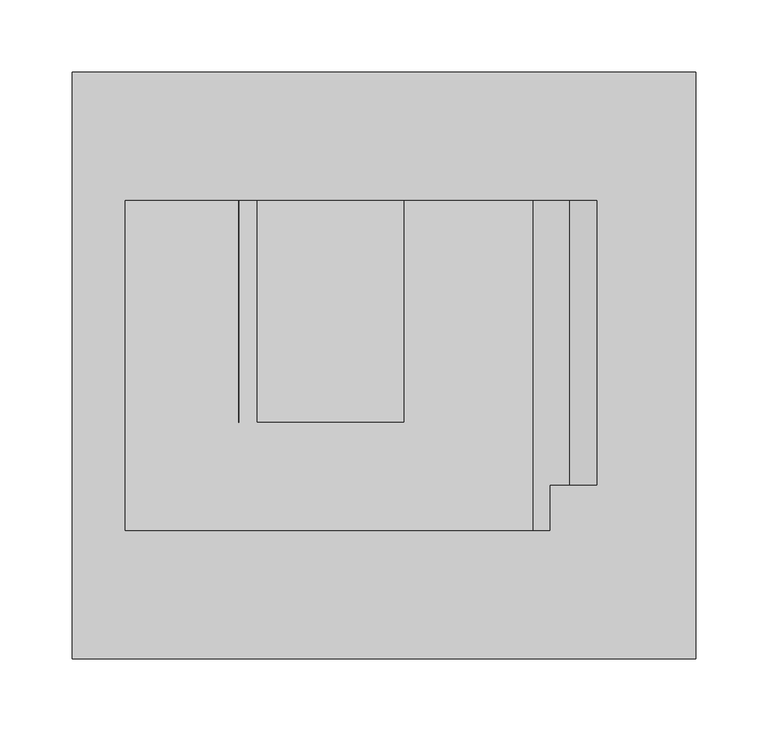
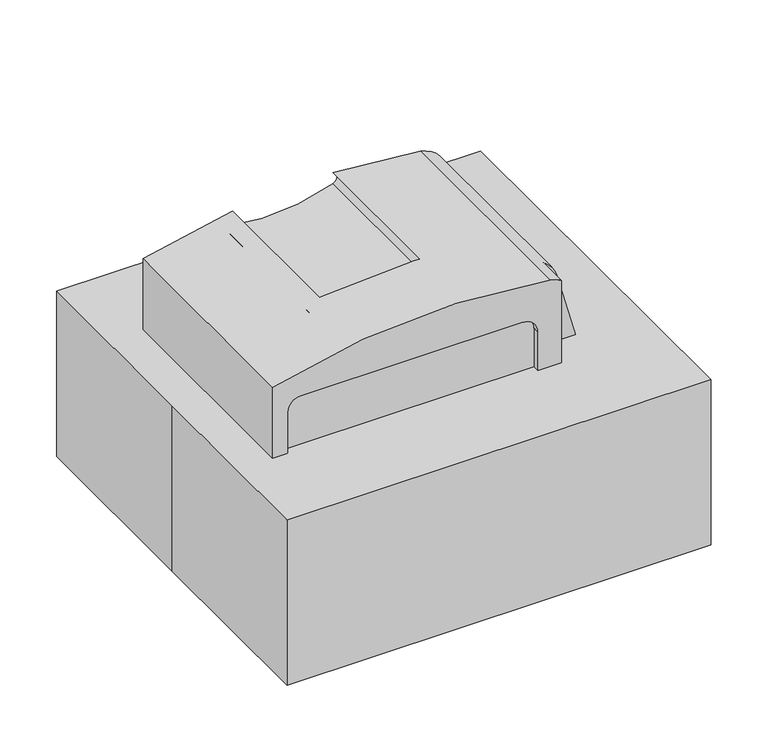
"""IFC4 building model written with IfcOpenShell, lengths in millimetres: proxy geometry, M7820 - Monitor, Fetal, Bedside-Stand Alone : M7820 - Monitor, Fetal, Bedside-Stand Alone."""

import ifcopenshell
import ifcopenshell.guid

model = None  # the IFC model being written
_history = None  # IfcOwnerHistory: only IFC2X3 demands one
_inside = {}  # id of a spatial element -> (the spatial element, [elements in it])
_under = {}  # id of a project, library or spatial element -> (it, [spatial elements below it])
_declared = {}  # id of a project -> (the project, [libraries it declares])
_typed = {}  # id of a type object -> (the type object, [elements of that type])
_made_of = {}  # id of a material, layer set ... -> (it, [elements and type objects made of it])


def new_model(schema):
    """Start an empty IFC model of exactly this schema.

    Asked for "IFC4X3", IfcOpenShell would pick the latest addendum, in which some entities
    have other attributes; the version numbers below select the first issue.
    IFC2X3 requires an IfcOwnerHistory on every rooted entity: one is made here for all.
    """
    global model, _history
    if schema == "IFC4X3":
        model = ifcopenshell.file(schema_version=(4, 3, 0, 0))
    else:
        model = ifcopenshell.file(schema=schema)
    _inside.clear()
    _under.clear()
    _declared.clear()
    _typed.clear()
    _made_of.clear()
    _history = None
    if model.schema == "IFC2X3":
        org = make("IfcOrganization", Name="unknown")
        user = make(
            "IfcPersonAndOrganization",
            ThePerson=make("IfcPerson", FamilyName="unknown"),
            TheOrganization=org,
        )
        app = make(
            "IfcApplication",
            ApplicationDeveloper=org,
            Version="unknown",
            ApplicationFullName="unknown",
            ApplicationIdentifier="unknown",
        )
        _history = make(
            "IfcOwnerHistory",
            OwningUser=user,
            OwningApplication=app,
            ChangeAction="ADDED",
            CreationDate=0,
        )
    return model


def make(cls, **values):
    """One entity of the class cls with the attributes given. An attribute that is None is left unset."""
    return model.create_entity(
        cls, **{name: value for name, value in values.items() if value is not None}
    )


def rooted(cls, **values):
    """An entity with a GlobalId (a new one), such as an element, a storey or a relation."""
    return make(cls, GlobalId=ifcopenshell.guid.new(), OwnerHistory=_history, **values)


def si_unit(unit_type, name, prefix=None):
    """IfcSIUnit, for example si_unit("LENGTHUNIT", "METRE", prefix="MILLI")."""
    return make("IfcSIUnit", UnitType=unit_type, Prefix=prefix, Name=name)


def assignment(units):
    """IfcUnitAssignment: the units of a project."""
    return None if units is None else make("IfcUnitAssignment", Units=units)


def point(xyz):
    """IfcCartesianPoint."""
    return None if xyz is None else make("IfcCartesianPoint", Coordinates=xyz)


def direction(xyz):
    """IfcDirection."""
    return None if xyz is None else make("IfcDirection", DirectionRatios=xyz)


def frame(location, z_axis=None, x_axis=None):
    """IfcAxis2Placement3D, a coordinate frame: its origin and axes. An axis left out is left unset."""
    return make(
        "IfcAxis2Placement3D",
        Location=point(location),
        Axis=direction(z_axis),
        RefDirection=direction(x_axis),
    )


def origin():
    """The frame at (0, 0, 0) with its axes left unset."""
    return frame((0.0, 0.0, 0.0))


def origin_with_axes():
    """The frame at (0, 0, 0) with the z axis (0, 0, 1) and the x axis (1, 0, 0) written out."""
    return frame((0.0, 0.0, 0.0), z_axis=(0.0, 0.0, 1.0), x_axis=(1.0, 0.0, 0.0))


def place(relative_to, where):
    """IfcLocalPlacement: puts the frame where relative to a parent placement (None: the world)."""
    return make(
        "IfcLocalPlacement", PlacementRelTo=relative_to, RelativePlacement=where
    )


def context(
    kind, dimensions, precision=None, world=None, true_north=None, identifier=None
):
    """IfcGeometricRepresentationContext, for example the 3D "Model" context."""
    return make(
        "IfcGeometricRepresentationContext",
        ContextIdentifier=identifier,
        ContextType=kind,
        CoordinateSpaceDimension=dimensions,
        Precision=precision,
        WorldCoordinateSystem=world,
        TrueNorth=true_north,
    )


def project(units=None, contexts=None):
    """IfcProject with its units and contexts."""
    return rooted(
        "IfcProject",
        Name="project",
        RepresentationContexts=contexts,
        UnitsInContext=assignment(units),
    )


def spatial(cls, under=None, at=None, **own):
    """A site, building, storey or space (cls), placed at a placement, below another one or the project."""
    s = rooted(cls, ObjectPlacement=at, **own)
    if under is not None:
        _under.setdefault(under.id(), (under, []))[1].append(s)
    return s


def polyline(points):
    """IfcPolyline through the points."""
    return make("IfcPolyline", Points=[point(p) for p in points])


def circle_curve(where, radius):
    """IfcCircle in the frame where."""
    return make("IfcCircle", Position=where, Radius=radius)


def outline(outer, holes=None, kind="AREA"):
    """IfcArbitraryClosedProfileDef: a profile drawn as a closed curve; with holes, ...WithVoids."""
    if holes is None:
        return make("IfcArbitraryClosedProfileDef", ProfileType=kind, OuterCurve=outer)
    return make(
        "IfcArbitraryProfileDefWithVoids",
        ProfileType=kind,
        OuterCurve=outer,
        InnerCurves=holes,
    )


def extrude(swept, where, along, depth):
    """IfcExtrudedAreaSolid: the profile swept, set in the frame where, extruded along a direction by depth."""
    return make(
        "IfcExtrudedAreaSolid",
        SweptArea=swept,
        Position=where,
        ExtrudedDirection=direction(along),
        Depth=depth,
    )


def shape(context_of_items, identifier, shape_type, items):
    """IfcShapeRepresentation: the items that make up one representation, for example the "Body"."""
    return make(
        "IfcShapeRepresentation",
        ContextOfItems=context_of_items,
        RepresentationIdentifier=identifier,
        RepresentationType=shape_type,
        Items=items,
    )


def source(mapping_origin, context_of_items, identifier, shape_type, items):
    """IfcRepresentationMap: a shape defined once, which mapped items show again and again."""
    return make(
        "IfcRepresentationMap",
        MappingOrigin=mapping_origin,
        MappedRepresentation=shape(context_of_items, identifier, shape_type, items),
    )


def transform(
    local_origin,
    x_axis=None,
    y_axis=None,
    z_axis=None,
    scale=None,
    scale2=None,
    scale3=None,
    uniform=True,
):
    """IfcCartesianTransformationOperator3D, or its non-uniform kind. x_axis, y_axis, z_axis: its Axis1, 2, 3."""
    if uniform:
        return make(
            "IfcCartesianTransformationOperator3D",
            Axis1=direction(x_axis),
            Axis2=direction(y_axis),
            LocalOrigin=point(local_origin),
            Scale=scale,
            Axis3=direction(z_axis),
        )
    return make(
        "IfcCartesianTransformationOperator3DnonUniform",
        Axis1=direction(x_axis),
        Axis2=direction(y_axis),
        LocalOrigin=point(local_origin),
        Scale=scale,
        Axis3=direction(z_axis),
        Scale2=scale2,
        Scale3=scale3,
    )


def mapped(mapping_source, mapping_target):
    """IfcMappedItem: shows the shape of a source again, moved by a transform."""
    return make(
        "IfcMappedItem", MappingSource=mapping_source, MappingTarget=mapping_target
    )


def made_of(thing, what):
    """Note that an element or type object is made of a material, layer set ...; save() writes the relation."""
    if what is not None:
        _made_of.setdefault(what.id(), (what, []))[1].append(thing)
    return thing


def element(
    cls,
    number,
    at=None,
    inside=None,
    cuts=None,
    type_object=None,
    material=None,
    context=None,
    identifier="Body",
    shape_type=None,
    held_by="IfcProductDefinitionShape",
    body=None,
    shapes=None,
    **own,
):
    """One element of the class cls, such as IfcWall. Its Tag is "e" and its number.

    at: its placement. inside: the storey or other place that contains it. cuts: it is an
    opening in that element (IfcRelVoidsElement). A single representation is given by context,
    identifier, shape_type and body (its items); several are given by shapes. held_by: the class
    of the entity that holds the representations. save() writes the other relations.
    """
    e = rooted(cls, Tag="e%d" % number, ObjectPlacement=at, **own)
    if body is not None:
        shapes = [shape(context, identifier, shape_type, body)]
    if shapes is not None:
        e.Representation = make(held_by, Representations=shapes)
    if inside is not None:
        _inside.setdefault(inside.id(), (inside, []))[1].append(e)
    if cuts is not None:
        rooted(
            "IfcRelVoidsElement", RelatingBuildingElement=cuts, RelatedOpeningElement=e
        )
    if type_object is not None:
        _typed.setdefault(type_object.id(), (type_object, []))[1].append(e)
    return made_of(e, material)


def aggregate(whole, parts):
    """IfcRelAggregates: a whole, such as a stair, and the parts it consists of."""
    return rooted("IfcRelAggregates", RelatingObject=whole, RelatedObjects=parts)


def save(model, path):
    """Write the relations noted so far, then the file.

    IfcRelAggregates (storeys below a building ...), IfcRelContainedInSpatialStructure (elements
    in a storey), IfcRelDefinesByType, IfcRelAssociatesMaterial and IfcRelDeclares: one each for
    every whole, place, type object, material and project.
    """
    for whole, parts in _under.values():
        aggregate(whole, parts)
    for where, things in _inside.values():
        rooted(
            "IfcRelContainedInSpatialStructure",
            RelatedElements=things,
            RelatingStructure=where,
        )
    for kind, things in _typed.values():
        rooted("IfcRelDefinesByType", RelatedObjects=things, RelatingType=kind)
    for what, things in _made_of.values():
        rooted("IfcRelAssociatesMaterial", RelatedObjects=things, RelatingMaterial=what)
    for by, libraries in _declared.values():
        rooted("IfcRelDeclares", RelatingContext=by, RelatedDefinitions=libraries)
    model.write(path)


def plane_surface(at):
    """IfcPlane: the flat surface through the origin of the frame at, square to its z axis."""
    return make("IfcPlane", Position=at)


def cylinder_surface(at, radius):
    """IfcCylindricalSurface: all points at the distance radius from the z axis of the frame at."""
    return make("IfcCylindricalSurface", Position=at, Radius=radius)


def revolved_surface(curve, axis_point, axis_direction):
    """IfcSurfaceOfRevolution: the curve turned about the line through axis_point along axis_direction."""
    return make(
        "IfcSurfaceOfRevolution",
        SweptCurve=make("IfcArbitraryOpenProfileDef", ProfileType="CURVE", Curve=curve),
        AxisPosition=make("IfcAxis1Placement", Location=point(axis_point), Axis=direction(axis_direction)),
    )


def advanced_brep(points, edges, surfaces, faces):
    """IfcAdvancedBrep: a solid bounded by faces that lie on surfaces and meet in shared edges.

    An edge is (start, end): straight between two places in points (the first is 0);
    or (start, end, curve); or (start, end, curve, False) where it runs against its curve.
    A face is (place in surfaces, loops), or (place, loops, False) where it looks against
    its surface's normal. A loop lists edges by number (the first is 1), with a minus sign
    where the edge is run from its end to its start. The first loop is the outer one.
    """
    corners = [point(p) for p in points]
    vertices = [make("IfcVertexPoint", VertexGeometry=c) for c in corners]
    made = []
    for start, end, *more in edges:
        made.append(
            make(
                "IfcEdgeCurve",
                EdgeStart=vertices[start],
                EdgeEnd=vertices[end],
                EdgeGeometry=more[0] if more else make("IfcPolyline", Points=[corners[start], corners[end]]),
                SameSense=more[1] if len(more) > 1 else True,
            )
        )
    hull = []
    for where, loops, *sense in faces:
        bounds = []
        for j, loop in enumerate(loops):
            ring = [make("IfcOrientedEdge", EdgeElement=made[abs(k) - 1], Orientation=k > 0) for k in loop]
            bounds.append(
                make(
                    "IfcFaceOuterBound" if j == 0 else "IfcFaceBound",
                    Bound=make("IfcEdgeLoop", EdgeList=ring),
                    Orientation=True,
                )
            )
        hull.append(make("IfcAdvancedFace", Bounds=bounds, FaceSurface=surfaces[where], SameSense=sense[0] if sense else True))
    return make("IfcAdvancedBrep", Outer=make("IfcClosedShell", CfsFaces=hull))


def specialty_equipment_b503c85d(model_context):
    return source(origin(), model_context, "Body", "SolidModel", [
        advanced_brep(
        [(150.8577319, -114.3, 0.0), (176.2577319, -114.3, 69.7859265), (114.7370728, -114.3, 110.2857558), (114.7370728, -114.3, 266.3346257), (103.1784124, -114.3, 270.7054998), (-179.3422681, -114.3, 254.0), (-179.3422681, -114.3, 0.0), (90.7109247, -114.3, 50.6960895), (71.6609247, -114.3, 31.6460895), (-144.2390753, -114.3, 31.6460895), (-163.2890753, -114.3, 50.6960895), (-163.2890753, -114.3, 222.1460895), (-150.5890753, -114.3, 234.8460895), (74.9738905, -114.3, 234.8460895), (90.7109247, -114.3, 219.1090553), (145.1038176, -114.3, 50.8544827), (94.3038176, -114.3, 50.8544827), (132.4038176, -114.3, 50.8544827), (107.0038176, -114.3, 50.8544827), (150.8577319, 114.3, 0.0), (-179.3422681, 114.3, 0.0), (-179.3422681, 114.3, 254.0), (-87.9648551, 114.3, 273.4915168), (-95.67799, 114.3, 271.6963039), (-95.5402402, 114.3, 259.3309192), (14.3607442, 114.3, 267.2445882), (14.1153613, 114.3, 279.2069302), (103.1784124, 114.3, 270.7054998), (128.6105233, 114.3, 247.6077295), (176.2577319, 114.3, 69.7859265), (150.8577319, -82.9767893, 0.0), (176.2577319, -82.9767893, 69.7859265), (128.6105233, -82.9767893, 247.6077295), (114.7370728, -82.9767893, 266.3346257), (14.1153613, -39.4871687, 279.2069302), (-87.9648551, -39.4871687, 273.4915168), (14.3607442, -39.4871687, 267.2445882), (-95.5402402, -39.4871687, 259.3309192), (-95.67799, -39.4871687, 271.6963039), (71.6609247, -107.5167707, 31.6460895), (90.7109247, -107.5167707, 50.6960895), (90.7109247, -107.5167707, 219.1090553), (74.9738905, -107.5167707, 234.8460895), (-150.5890753, -107.5167707, 234.8460895), (-163.2890753, -107.5167707, 222.1460895), (-163.2890753, -107.5167707, 50.6960895), (-144.2390753, -107.5167707, 31.6460895), (94.3038176, -82.9767893, 50.8544827), (145.1038176, -82.9767893, 50.8544827), (107.0038176, -82.9767893, 50.8544827), (132.4038176, -82.9767893, 50.8544827), (114.7370728, -82.9767893, 110.2857558)],
        [
            (0, 1, circle_curve(frame((119.7038176, -114.3, 50.8544827), z_axis=(0.0, -1.0, 0.0), x_axis=(1.0, 0.0, 0.0)), 59.6384505)),
            (1, 2, circle_curve(frame((119.7038176, -114.3, 50.8544827), z_axis=(0.0, -1.0, 0.0), x_axis=(1.0, 0.0, 0.0)), 59.6384505)),
            (2, 3),
            (3, 4, circle_curve(frame((97.9423784, -114.3, 239.3902248), z_axis=(0.0, -1.0, 0.0), x_axis=(1.0, 0.0, 0.0)), 31.75)),
            (4, 5, circle_curve(frame((-1.5422681, -114.3, -355.6), z_axis=(0.0, -1.0, 0.0), x_axis=(1.0, 0.0, 0.0)), 635.0)),
            (5, 6),
            (6, 0),
            (7, 8, circle_curve(frame((71.6609247, -114.3, 50.6960895), z_axis=(0.0, 1.0, 0.0), x_axis=(1.0, 0.0, 0.0)), 19.05)),
            (8, 9),
            (9, 10, circle_curve(frame((-144.2390753, -114.3, 50.6960895), z_axis=(0.0, 1.0, 0.0), x_axis=(1.0, 0.0, 0.0)), 19.05)),
            (10, 11),
            (11, 12, circle_curve(frame((-150.5890753, -114.3, 222.1460895), z_axis=(0.0, 1.0, 0.0), x_axis=(1.0, 0.0, 0.0)), 12.7)),
            (12, 13),
            (13, 14, circle_curve(frame((74.9738905, -114.3, 219.1090553), z_axis=(0.0, 1.0, 0.0), x_axis=(1.0, 0.0, 0.0)), 15.7370342)),
            (14, 7),
            (15, 16, circle_curve(frame((119.7038176, -114.3, 50.8544827), z_axis=(0.0, 1.0, 0.0), x_axis=(1.0, 0.0, 0.0)), 25.4)),
            (16, 15, circle_curve(frame((119.7038176, -114.3, 50.8544827), z_axis=(0.0, 1.0, 0.0), x_axis=(1.0, 0.0, 0.0)), 25.4)),
            (17, 18, circle_curve(frame((119.7038176, -114.3, 50.8544827), z_axis=(0.0, -1.0, 0.0), x_axis=(1.0, 0.0, 0.0)), 12.7)),
            (18, 17, circle_curve(frame((119.7038176, -114.3, 50.8544827), z_axis=(0.0, -1.0, 0.0), x_axis=(1.0, 0.0, 0.0)), 12.7)),
            (19, 20),
            (20, 21),
            (21, 22, circle_curve(frame((-1.5422681, 114.3, -355.6), z_axis=(0.0, 1.0, 0.0), x_axis=(1.0, 0.0, 0.0)), 635.0)),
            (22, 23, circle_curve(frame((-18.6096514, 114.3, -41.9605774), z_axis=(0.0, -1.0, 0.0), x_axis=(1.0, 0.0, 0.0)), 322.9863279)),
            (23, 24, circle_curve(frame((-94.1628052, 114.3, 265.5297234), z_axis=(0.0, -1.0, 0.0), x_axis=(1.0, 0.0, 0.0)), 6.35)),
            (24, 25, circle_curve(frame((-53.8232511, 114.3, 447.0678714), z_axis=(0.0, -1.0, 0.0), x_axis=(1.0, 0.0, 0.0)), 192.316069)),
            (25, 26, circle_curve(frame((12.1094067, 114.3, 273.1820944), z_axis=(0.0, -1.0, 0.0), x_axis=(1.0, 0.0, 0.0)), 6.35)),
            (26, 27, circle_curve(frame((-1.5422681, 114.3, -355.6), z_axis=(0.0, 1.0, 0.0), x_axis=(1.0, 0.0, 0.0)), 635.0)),
            (27, 28, circle_curve(frame((97.9423784, 114.3, 239.3902248), z_axis=(0.0, 1.0, 0.0), x_axis=(1.0, 0.0, 0.0)), 31.75)),
            (28, 29),
            (29, 19, circle_curve(frame((119.7038176, 114.3, 50.8544827), z_axis=(0.0, 1.0, 0.0), x_axis=(1.0, 0.0, 0.0)), 59.6384505)),
            (0, 30),
            (30, 19),
            (29, 31),
            (31, 1),
            (28, 32),
            (32, 31),
            (27, 4),
            (3, 33),
            (33, 32, circle_curve(frame((97.9423784, -82.9767893, 239.3902248), z_axis=(0.0, 1.0, 0.0), x_axis=(1.0, 0.0, 0.0)), 31.75)),
            (26, 34),
            (34, 35, circle_curve(frame((-1.5422681, -39.4871687, -355.6), z_axis=(0.0, -1.0, 0.0), x_axis=(1.0, 0.0, 0.0)), 635.0)),
            (35, 22),
            (21, 5),
            (20, 6),
            (36, 37, circle_curve(frame((-53.8232511, -39.4871687, 447.0678714), z_axis=(0.0, 1.0, 0.0), x_axis=(1.0, 0.0, 0.0)), 192.316069)),
            (37, 38, circle_curve(frame((-94.1628052, -39.4871687, 265.5297234), z_axis=(0.0, 1.0, 0.0), x_axis=(1.0, 0.0, 0.0)), 6.35)),
            (38, 35, circle_curve(frame((-18.6096514, -39.4871687, -41.9605774), z_axis=(0.0, 1.0, 0.0), x_axis=(1.0, 0.0, 0.0)), 322.9863279)),
            (34, 36, circle_curve(frame((12.1094067, -39.4871687, 273.1820944), z_axis=(0.0, 1.0, 0.0), x_axis=(1.0, 0.0, 0.0)), 6.35)),
            (25, 36),
            (38, 23),
            (37, 24),
            (39, 40, circle_curve(frame((71.6609247, -107.5167707, 50.6960895), z_axis=(0.0, -1.0, 0.0), x_axis=(1.0, 0.0, 0.0)), 19.05)),
            (40, 41),
            (41, 42, circle_curve(frame((74.9738905, -107.5167707, 219.1090553), z_axis=(0.0, -1.0, 0.0), x_axis=(1.0, 0.0, 0.0)), 15.7370342)),
            (42, 43),
            (43, 44, circle_curve(frame((-150.5890753, -107.5167707, 222.1460895), z_axis=(0.0, -1.0, 0.0), x_axis=(1.0, 0.0, 0.0)), 12.7)),
            (44, 45),
            (45, 46, circle_curve(frame((-144.2390753, -107.5167707, 50.6960895), z_axis=(0.0, -1.0, 0.0), x_axis=(1.0, 0.0, 0.0)), 19.05)),
            (46, 39),
            (39, 8),
            (7, 40),
            (14, 41),
            (13, 42),
            (12, 43),
            (11, 44),
            (10, 45),
            (9, 46),
            (47, 48, circle_curve(frame((119.7038176, -82.9767893, 50.8544827), z_axis=(0.0, -1.0, 0.0), x_axis=(1.0, 0.0, 0.0)), 25.4)),
            (48, 47, circle_curve(frame((119.7038176, -82.9767893, 50.8544827), z_axis=(0.0, -1.0, 0.0), x_axis=(1.0, 0.0, 0.0)), 25.4)),
            (49, 50, circle_curve(frame((119.7038176, -82.9767893, 50.8544827), z_axis=(0.0, 1.0, 0.0), x_axis=(1.0, 0.0, 0.0)), 12.7)),
            (50, 49, circle_curve(frame((119.7038176, -82.9767893, 50.8544827), z_axis=(0.0, 1.0, 0.0), x_axis=(1.0, 0.0, 0.0)), 12.7)),
            (51, 31, circle_curve(frame((119.7038176, -82.9767893, 50.8544827), z_axis=(0.0, 1.0, 0.0), x_axis=(1.0, 0.0, 0.0)), 59.6384505)),
            (33, 51),
            (51, 2),
            (47, 16),
            (15, 48),
            (49, 18),
            (17, 50),
        ],
        [
            plane_surface(frame((179.3422681, -114.3, 50.8544827), z_axis=(0.0, -1.0, 0.0), x_axis=(0.0, 0.0, 1.0))),
            plane_surface(frame((179.3422681, 114.3, 50.8544827), z_axis=(0.0, 1.0, 0.0), x_axis=(0.0, 0.0, -1.0))),
            cylinder_surface(frame((119.7038176, 114.3, 50.8544827), z_axis=(0.0, -1.0, 0.0), x_axis=(1.0, 0.0, 0.0)), 59.6384505),
            plane_surface(frame((176.2577319, -114.3, 69.7859265), z_axis=(0.9659258262890688, 0.0, 0.25881904510251935), x_axis=(0.0, 1.0, 0.0))),
            cylinder_surface(frame((97.9423784, 114.3, 239.3902248), z_axis=(0.0, -1.0, 0.0), x_axis=(1.0, 0.0, 0.0)), 31.75),
            cylinder_surface(frame((-1.5422681, 114.3, -355.6), z_axis=(0.0, -1.0, 0.0), x_axis=(1.0, 0.0, 0.0)), 635.0),
            plane_surface(frame((-179.3422681, -114.3, 254.0), z_axis=(-1.0, 0.0, 0.0), x_axis=(0.0, 1.0, 0.0))),
            plane_surface(frame((-179.3422681, -114.3, 0.0), z_axis=(0.0, 0.0, -1.0), x_axis=(0.0, 1.0, 0.0))),
            plane_surface(frame((18.4594067, -39.4871687, 273.1820944), z_axis=(0.0, 1.0, 0.0), x_axis=(0.0, 0.0, 1.0))),
            revolved_surface(polyline([(18.4594067, -39.4871687, 273.1820944), (18.4594067, 114.3, 273.1820944)]), (12.1094067, 114.3, 273.1820944), (0.0, -1.0, 0.0)),
            revolved_surface(polyline([(304.3766765, -39.4871687, -41.9605774), (304.3766765, 114.3, -41.9605774)]), (-18.6096514, 114.3, -41.9605774), (0.0, -1.0, 0.0)),
            revolved_surface(polyline([(-87.8128052, -39.4871687, 265.5297234), (-87.8128052, 114.3, 265.5297234)]), (-94.1628052, 114.3, 265.5297234), (0.0, -1.0, 0.0)),
            revolved_surface(polyline([(138.4928179, -39.4871687, 447.0678714), (138.4928179, 114.3, 447.0678714)]), (-53.8232511, 114.3, 447.0678714), (0.0, -1.0, 0.0)),
            plane_surface(frame((90.7109247, -107.5167707, 50.6960895), z_axis=(0.0, -1.0, 0.0), x_axis=(0.0, 0.0, -1.0))),
            revolved_surface(polyline([(90.71092469999999, -114.3, 50.6960895), (90.71092469999999, -107.5167707, 50.6960895)]), (71.6609247, -107.5167707, 50.6960895), (0.0, -1.0, 0.0)),
            plane_surface(frame((90.7109247, -114.3, 50.6960895), z_axis=(-1.0, 0.0, 0.0), x_axis=(0.0, 1.0, 0.0))),
            revolved_surface(polyline([(90.71092469999999, -114.3, 219.1090553), (90.71092469999999, -107.5167707, 219.1090553)]), (74.9738905, -107.5167707, 219.1090553), (0.0, -1.0, 0.0)),
            plane_surface(frame((74.9738905, -114.3, 234.8460895), z_axis=(0.0, 0.0, -1.0), x_axis=(0.0, 1.0, 0.0))),
            revolved_surface(polyline([(-137.8890753, -114.3, 222.1460895), (-137.8890753, -107.5167707, 222.1460895)]), (-150.5890753, -107.5167707, 222.1460895), (0.0, -1.0, 0.0)),
            plane_surface(frame((-163.2890753, -114.3, 222.1460895), z_axis=(1.0, 0.0, 0.0), x_axis=(0.0, 1.0, 0.0))),
            revolved_surface(polyline([(-125.1890753, -114.3, 50.6960895), (-125.1890753, -107.5167707, 50.6960895)]), (-144.2390753, -107.5167707, 50.6960895), (0.0, -1.0, 0.0)),
            plane_surface(frame((-144.2390753, -114.3, 31.6460895), z_axis=(0.0, 0.0, 1.0), x_axis=(0.0, 1.0, 0.0))),
            plane_surface(frame((179.3422681, -82.9767893, 50.8544827), z_axis=(0.0, -1.0, 0.0), x_axis=(0.0, 0.0, 1.0))),
            cylinder_surface(frame((119.7038176, -82.9767893, 50.8544827), z_axis=(0.0, 1.0, 0.0), x_axis=(1.0, 0.0, 0.0)), 59.6384505),
            plane_surface(frame((114.7370728, -114.3, 288.0857558), z_axis=(1.0, 0.0, 0.0), x_axis=(0.0, 1.0, 0.0))),
            revolved_surface(polyline([(145.10381759999999, -114.3, 50.8544827), (145.10381759999999, -82.9767893, 50.8544827)]), (119.7038176, 114.3, 50.8544827), (0.0, -1.0, 0.0)),
            cylinder_surface(frame((119.7038176, 114.3, 50.8544827), z_axis=(0.0, 1.0, 0.0), x_axis=(1.0, 0.0, 0.0)), 12.7),
        ],
        [
            (0, [[1, 2, 3, 4, 5, 6, 7], [8, 9, 10, 11, 12, 13, 14, 15], [16, 17]]),
            (0, [[18, 19]]),
            (1, [[20, 21, 22, 23, 24, 25, 26, 27, 28, 29, 30]]),
            (2, [[-1, 31, 32, -30, 33, 34]]),
            (3, [[-29, 35, 36, -33]]),
            (4, [[-28, 37, -4, 38, 39, -35]]),
            (5, [[-5, -37, -27, 40, 41, 42, -22, 43]]),
            (6, [[-6, -43, -21, 44]]),
            (7, [[-7, -44, -20, -32, -31]]),
            (8, [[45, 46, 47, -41, 48]]),
            (9, [[49, -48, -40, -26]]),
            (10, [[50, -23, -42, -47]]),
            (11, [[-46, 51, -24, -50]]),
            (12, [[-45, -49, -25, -51]]),
            (13, [[52, 53, 54, 55, 56, 57, 58, 59]]),
            (14, [[-52, 60, -8, 61]]),
            (15, [[-53, -61, -15, 62]]),
            (16, [[-54, -62, -14, 63]]),
            (17, [[-55, -63, -13, 64]]),
            (18, [[-56, -64, -12, 65]]),
            (19, [[-57, -65, -11, 66]]),
            (20, [[-58, -66, -10, 67]]),
            (21, [[-59, -67, -9, -60]]),
            (22, [[68, 69], [70, 71]]),
            (22, [[72, -36, -39, 73]]),
            (23, [[74, -2, -34, -72]]),
            (24, [[-74, -73, -38, -3]]),
            (25, [[-68, 75, -16, 76]]),
            (25, [[-69, -76, -17, -75]]),
            (26, [[-70, 77, -18, 78]]),
            (26, [[-71, -78, -19, -77]]),
        ],
    ),
        extrude(outline(polyline([(-215.9, 203.2), (215.9, 203.2), (215.9, -203.2), (-215.9, -203.2), (-215.9, 0.0), (-215.9, 203.2)])), origin_with_axes(), (0.0, 0.0, 1.0), 177.8),
    ])


if __name__ == "__main__":
    model = new_model("IFC4")
    model_context = context("Model", 3, world=origin())
    ifc_project = project(units=[si_unit("LENGTHUNIT", "METRE", prefix="MILLI")], contexts=[model_context])
    site = spatial("IfcSite", under=ifc_project)
    building = spatial("IfcBuilding", under=site)
    placement = place(None, origin())
    specialty_equipment_shape = specialty_equipment_b503c85d(model_context)
    element("IfcBuildingElementProxy", 1, Name="M7820 - Monitor, Fetal, Bedside-Stand Alone : M7820 - Monitor, Fetal, Bedside-Stand Alone", ObjectType="M7820 - Monitor, Fetal, Bedside-Stand Alone : M7820 - Monitor, Fetal, Bedside-Stand Alone", at=placement, inside=building, context=model_context, shape_type="MappedRepresentation", body=[
        mapped(specialty_equipment_shape, transform((0.0, 0.0, 0.0), x_axis=(1.0, 0.0, 0.0), y_axis=(0.0, 1.0, 0.0), z_axis=(0.0, 0.0, 1.0))),
    ])
    save(model, "model.ifc")

# Revit data of these elements
# Project information
#   Sheets - Total = "6"
#   Project Issue Date = "Issue Date"
#   Project Status = "Project Status"
#   Client Name = "Owner"
#   Project Address = "Enter address here"
#   Project Name = "Project Name"
#   Project Number = "Project Number"
#   Publication Date = "30-Jan-15"
# Type "M7820 - Monitor, Fetal, Bedside-Stand Alone : M7820 - Monitor, Fetal, Bedside-Stand Alone"
#   Watts2 = "0"
#   Watts1 = "120"
#   Unit_Issue = "EA"
#   UTIL_6_Misc = "D"
#   UTIL_5_NonMedGas = "-"
#   UTIL_4_MiscGas = "-"
#   UTIL_3_MedGas = "-"
#   UTIL_2_Elec = "A"
#   UTIL_1_WaterDrain = "-"
#   Nomenclature = "Monitor, Fetal, Bedside/Stand Alone"
#   NSN = "6515"
#   Location [instance default] = ""
#   JSN = "M7820"
#   Fund_Source_VA = "-"
#   Fund_Source_Navy = "-"
#   Fund_Source_Army = "-"
#   Fund_Source_AF = "-"
#   ELEC_Volts2 = "0"
#   ELEC_Volts1 = "120"
#   ELEC_Phase2 = "0"
#   ELEC_Phase1 = "1"
#   ELEC_HertzSwitch = "0"
#   ELEC_HertzDependent = "-1"
#   ELEC_Hertz = "60"
#   ELEC_Amps2 = "0"
#   ELEC_Amps1 = "1"
#   DetailDescription = "Bedside fetal monitor. May be stand alone or connected to a central monitoring station. It includes dual heart rate, direct fetal ECG and ultrasound methods for monitoring fetal heart rate, it also monitors uterine activity. It has a 2 channel recording mechanisms with automatic annotation and a highly sensitive Doppler. Unit has telephone transmission capabilities. Used to monitor and evaluate contractions ante-partum."
#   CAT_VA = "C"
#   CAT_Navy = "C"
#   CAT_IHS = "-"
#   CAT_Army = "C"
#   CAT_AF = "C"
#   BTUperhour = "0"
#   Weight_IP = 32
#   DIM_Width_IP = 1' - 5"
#   DIM_Height_IP = 0' - 7"
#   DIM_Depth_IP = 1' - 4"
#   finish [instance default] = none
# Element 1 (IfcBuildingElementProxy, "M7820 - Monitor, Fetal, Bedside-Stand Alone : M7820 - Monitor, Fetal, Bedside-Stand Alone")
#   Materials on its faces: "EquipSpace"
# Materials
#   "EquipSpace": class "Unassigned", colour RGB 221 217 195, transparency 0.5
